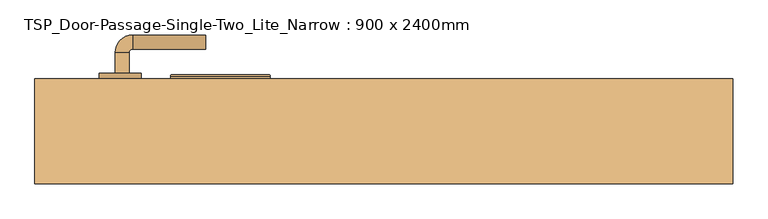
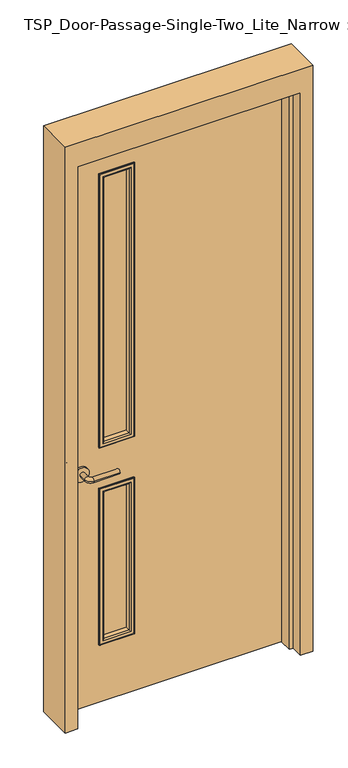
"""IFC4 building model written with IfcOpenShell, lengths in millimetres: door geometry, TSP_Door-Passage-Single-Two_Lite_Narrow : 900 x 2400mm."""

from ifc_helpers import new_model, si_unit, point, frame, frame_2d, origin, place, context, project, spatial, polyline, circle_curve, ellipse_curve, trimmed, segment, composite_curve, outline, extrude, faceted_brep, source, transform, mapped, element, save
from ifc_brep_helpers import plane_surface, cylinder_surface, revolved_surface, advanced_brep


def tsp_door_passage_single_two_lite_narrow_900_x_2400mm_46d0a56f(model_context):
    return source(origin(), model_context, "Body", "SolidModel", [
        advanced_brep(
        [(-384.990625, 48.35, 1000.0), (-364.990625, 48.35, 1000.0), (-364.990625, 18.35, 1000.0), (-384.990625, 18.35, 1000.0), (-359.990625, 13.35, 1000.0), (-359.990625, -6.65, 1000.0), (-254.990625, -6.65, 1000.0), (-254.990625, 13.35, 1000.0)],
        [
            (0, 1, circle_curve(frame((-374.990625, 48.35, 1000.0), z_axis=(0.0, 1.0, 0.0), x_axis=(1.0, 0.0, 0.0)), 10.0)),
            (1, 0, circle_curve(frame((-374.990625, 48.35, 1000.0), z_axis=(0.0, 1.0, 0.0), x_axis=(1.0, 0.0, 0.0)), 10.0)),
            (1, 2),
            (2, 3, circle_curve(frame((-374.990625, 18.35, 1000.0), z_axis=(0.0, 1.0, 0.0), x_axis=(1.0, 0.0, 0.0)), 10.0)),
            (3, 0),
            (3, 2, circle_curve(frame((-374.990625, 18.35, 1000.0), z_axis=(0.0, 1.0, 0.0), x_axis=(1.0, 0.0, 0.0)), 10.0)),
            (4, 5, circle_curve(frame((-359.990625, 3.35, 1000.0), z_axis=(-1.0, 0.0, 0.0), x_axis=(0.0, 1.0, 0.0)), 10.0)),
            (5, 3, circle_curve(frame((-359.990625, 18.35, 1000.0), z_axis=(0.0, 0.0, -1.0), x_axis=(-1.0, 0.0, 0.0)), 25.0)),
            (2, 4, circle_curve(frame((-359.990625, 18.35, 1000.0), z_axis=(0.0, 0.0, 1.0), x_axis=(-1.0, 0.0, 0.0)), 5.0)),
            (5, 4, circle_curve(frame((-359.990625, 3.35, 1000.0), z_axis=(-1.0, 0.0, 0.0), x_axis=(0.0, 1.0, 0.0)), 10.0)),
            (6, 7, circle_curve(frame((-254.990625, 3.35, 1000.0), z_axis=(1.0, 0.0, 0.0), x_axis=(0.0, 1.0, 0.0)), 10.0)),
            (7, 6, circle_curve(frame((-254.990625, 3.35, 1000.0), z_axis=(1.0, 0.0, 0.0), x_axis=(0.0, 1.0, 0.0)), 10.0)),
            (4, 7),
            (6, 5),
        ],
        [
            plane_surface(frame((-374.990625, 48.35, 1000.0), z_axis=(0.0, 1.0, 0.0), x_axis=(0.0, 0.0, 1.0))),
            cylinder_surface(frame((-374.990625, 48.35, 1000.0), z_axis=(0.0, 1.0, 0.0), x_axis=(1.0, 0.0, 0.0)), 10.0),
            revolved_surface(trimmed(ellipse_curve(frame((-374.990625, 18.35, 1000.0), z_axis=(0.0, -1.0, 0.0), x_axis=(1.0, 0.0, 0.0)), 10.0, 10.0), [point((-384.990625, 18.35, 1000.0))], [point((-364.990625, 18.35, 1000.0))], True, "CARTESIAN"), (-359.990625, 18.35, 1000.0), (0.0, 0.0, -1.0)),
            revolved_surface(trimmed(ellipse_curve(frame((-374.990625, 18.35, 1000.0), z_axis=(0.0, -1.0, 0.0), x_axis=(1.0, 0.0, 0.0)), 10.0, 10.0), [point((-364.990625, 18.35, 1000.0))], [point((-384.990625, 18.35, 1000.0))], True, "CARTESIAN"), (-359.990625, 18.35, 1000.0), (0.0, 0.0, -1.0)),
            plane_surface(frame((-254.990625, 3.35, 1000.0), z_axis=(1.0, 0.0, 0.0), x_axis=(0.0, 0.0, 1.0))),
            cylinder_surface(frame((-359.990625, 3.35, 1000.0), z_axis=(-1.0, 0.0, 0.0), x_axis=(0.0, 1.0, 0.0)), 10.0),
        ],
        [
            (0, [[1, 2]]),
            (1, [[3, 4, 5, -2]]),
            (1, [[-5, 6, -3, -1]]),
            (2, [[7, 8, -4, 9]]),
            (3, [[10, -9, -6, -8]]),
            (4, [[11, 12]]),
            (5, [[13, -11, 14, -7]]),
            (5, [[-14, -12, -13, -10]]),
        ],
    ),
        extrude(outline(composite_curve([segment(trimmed(circle_curve(frame_2d((1000.0, -377.490625)), 30.0), [point((1000.0, -407.490625))], [point((1000.0, -347.490625))], False, "CARTESIAN"), True, "CONTINUOUS"), segment(trimmed(circle_curve(frame_2d((1000.0, -377.490625)), 30.0), [point((1000.0, -347.490625))], [point((1000.0, -407.490625))], False, "CARTESIAN"), True, "CONTINUOUS")], self_intersect=False)), frame((0.0, 48.35, 0.0), z_axis=(0.0, 1.0, 0.0), x_axis=(0.0, 0.0, 1.0)), (0.0, 0.0, 1.0), 8.0),
        advanced_brep(
        [(-384.990625, 109.35, 1000.0), (-364.990625, 109.35, 1000.0), (-384.990625, 139.35, 1000.0), (-364.990625, 139.35, 1000.0), (-359.990625, 144.35, 1000.0), (-359.990625, 164.35, 1000.0), (-254.990625, 164.35, 1000.0), (-254.990625, 144.35, 1000.0)],
        [
            (0, 1, circle_curve(frame((-374.990625, 109.35, 1000.0), z_axis=(0.0, -1.0, 0.0), x_axis=(1.0, 0.0, 0.0)), 10.0)),
            (1, 0, circle_curve(frame((-374.990625, 109.35, 1000.0), z_axis=(0.0, -1.0, 0.0), x_axis=(1.0, 0.0, 0.0)), 10.0)),
            (0, 2),
            (2, 3, circle_curve(frame((-374.990625, 139.35, 1000.0), z_axis=(0.0, -1.0, 0.0), x_axis=(1.0, 0.0, 0.0)), 10.0)),
            (3, 1),
            (3, 2, circle_curve(frame((-374.990625, 139.35, 1000.0), z_axis=(0.0, -1.0, 0.0), x_axis=(1.0, 0.0, 0.0)), 10.0)),
            (4, 3, circle_curve(frame((-359.990625, 139.35, 1000.0), z_axis=(0.0, 0.0, 1.0), x_axis=(-1.0, 0.0, 0.0)), 5.0)),
            (2, 5, circle_curve(frame((-359.990625, 139.35, 1000.0), z_axis=(0.0, 0.0, -1.0), x_axis=(-1.0, 0.0, 0.0)), 25.0)),
            (5, 4, circle_curve(frame((-359.990625, 154.35, 1000.0), z_axis=(-1.0, 0.0, 0.0), x_axis=(0.0, -1.0, 0.0)), 10.0)),
            (4, 5, circle_curve(frame((-359.990625, 154.35, 1000.0), z_axis=(-1.0, 0.0, 0.0), x_axis=(0.0, -1.0, 0.0)), 10.0)),
            (6, 7, circle_curve(frame((-254.990625, 154.35, 1000.0), z_axis=(1.0, 0.0, 0.0), x_axis=(0.0, -1.0, 0.0)), 10.0)),
            (7, 6, circle_curve(frame((-254.990625, 154.35, 1000.0), z_axis=(1.0, 0.0, 0.0), x_axis=(0.0, -1.0, 0.0)), 10.0)),
            (5, 6),
            (7, 4),
        ],
        [
            plane_surface(frame((-374.990625, 109.35, 1000.0), z_axis=(0.0, -1.0, 0.0), x_axis=(0.0, 0.0, 1.0))),
            cylinder_surface(frame((-374.990625, 109.35, 1000.0), z_axis=(0.0, -1.0, 0.0), x_axis=(1.0, 0.0, 0.0)), 10.0),
            revolved_surface(trimmed(ellipse_curve(frame((-374.990625, 139.35, 1000.0), z_axis=(0.0, -1.0, 0.0), x_axis=(1.0, 0.0, 0.0)), 10.0, 10.0), [point((-384.990625, 139.35, 1000.0))], [point((-364.990625, 139.35, 1000.0))], True, "CARTESIAN"), (-359.990625, 139.35, 1000.0), (0.0, 0.0, -1.0)),
            revolved_surface(trimmed(ellipse_curve(frame((-374.990625, 139.35, 1000.0), z_axis=(0.0, -1.0, 0.0), x_axis=(1.0, 0.0, 0.0)), 10.0, 10.0), [point((-364.990625, 139.35, 1000.0))], [point((-384.990625, 139.35, 1000.0))], True, "CARTESIAN"), (-359.990625, 139.35, 1000.0), (0.0, 0.0, -1.0)),
            plane_surface(frame((-254.990625, 154.35, 1000.0), z_axis=(1.0, 0.0, 0.0), x_axis=(0.0, 0.0, 1.0))),
            cylinder_surface(frame((-359.990625, 154.35, 1000.0), z_axis=(-1.0, 0.0, 0.0), x_axis=(0.0, -1.0, 0.0)), 10.0),
        ],
        [
            (0, [[1, 2]]),
            (1, [[-1, 3, 4, 5]]),
            (1, [[-2, -5, 6, -3]]),
            (2, [[7, -4, 8, 9]]),
            (3, [[-8, -6, -7, 10]]),
            (4, [[11, 12]]),
            (5, [[-9, 13, -12, 14]]),
            (5, [[-10, -14, -11, -13]]),
        ],
    ),
        extrude(outline(composite_curve([segment(trimmed(circle_curve(frame_2d((1000.0, -377.490625)), 30.0), [point((1000.0, -407.490625))], [point((1000.0, -347.490625))], False, "CARTESIAN"), True, "CONTINUOUS"), segment(trimmed(circle_curve(frame_2d((1000.0, -377.490625)), 30.0), [point((1000.0, -347.490625))], [point((1000.0, -407.490625))], False, "CARTESIAN"), True, "CONTINUOUS")], self_intersect=False)), frame((0.0, 101.35, 0.0), z_axis=(0.0, 1.0, 0.0), x_axis=(0.0, 0.0, 1.0)), (0.0, 0.0, 1.0), 8.0),
        extrude(outline(polyline([(2400.0, -450.0), (0.0, -450.0), (0.0, 450.0), (2400.0, 450.0), (2400.0, -450.0)]), holes=[polyline([(2247.6, -297.6), (2247.6, -170.6), (1095.25, -170.6), (1095.25, -297.6), (2247.6, -297.6)]), polyline([(904.75, -297.6), (904.75, -170.6), (254.0, -170.6), (254.0, -297.6), (904.75, -297.6)])]), frame((0.0, 56.35, 0.0), z_axis=(0.0, 1.0, 0.0), x_axis=(0.0, 0.0, 1.0)), (0.0, 0.0, 1.0), 45.0),
        faceted_brep([(450.0, 51.5875, 0.0), (450.0, 101.35, 0.0), (500.0, 101.35, 0.0), (500.0, -48.65, 0.0), (450.0, -48.65, 0.0), (450.0, 0.5625, 0.0), (434.125, 0.5625, 0.0), (434.125, 51.5875, 0.0), (450.0, 51.5875, 2400.0), (450.0, 101.35, 2400.0), (-450.0, 101.35, 2400.0), (-450.0, 101.35, 0.0), (-500.0, 101.35, 0.0), (-500.0, 101.35, 2500.0), (500.0, 101.35, 2500.0), (500.0, -48.65, 2500.0), (-500.0, -48.65, 2500.0), (-500.0, -48.65, 0.0), (-450.0, -48.65, 0.0), (-450.0, -48.65, 2400.0), (450.0, -48.65, 2400.0), (450.0, 0.5625, 2400.0), (-450.0, 0.5625, 2400.0), (-450.0, 0.5625, 0.0), (-434.125, 0.5625, 0.0), (-434.125, 0.5625, 2384.125), (434.125, 0.5625, 2384.125), (434.125, 51.5875, 2384.125), (-434.125, 51.5875, 2384.125), (-434.125, 51.5875, 0.0), (-450.0, 51.5875, 0.0), (-450.0, 51.5875, 2400.0)], [[[0, 1, 2, 3, 4, 5, 6, 7]], [[1, 0, 8, 9]], [[2, 1, 9, 10, 11, 12, 13, 14]], [[3, 2, 14, 15]], [[4, 3, 15, 16, 17, 18, 19, 20]], [[5, 4, 20, 21]], [[6, 5, 21, 22, 23, 24, 25, 26]], [[7, 6, 26, 27]], [[0, 7, 27, 28, 29, 30, 31, 8]], [[9, 8, 31, 10]], [[20, 19, 22, 21]], [[26, 25, 28, 27]], [[12, 11, 30, 29, 24, 23, 18, 17]], [[11, 10, 31, 30]], [[13, 12, 17, 16]], [[19, 18, 23, 22]], [[25, 24, 29, 28]], [[15, 14, 13, 16]]]),
        extrude(outline(polyline([(-170.6, 75.675), (-297.6, 75.675), (-297.6, 82.025), (-170.6, 82.025), (-170.6, 75.675)])), frame((0.0, 0.0, 1095.25), z_axis=(0.0, 0.0, 1.0), x_axis=(1.0, 0.0, 0.0)), (0.0, 0.0, 1.0), 1152.35),
        extrude(outline(polyline([(-170.6, 75.675), (-297.6, 75.675), (-297.6, 82.025), (-170.6, 82.025), (-170.6, 75.675)])), frame((0.0, 0.0, 254.0), z_axis=(0.0, 0.0, 1.0), x_axis=(1.0, 0.0, 0.0)), (0.0, 0.0, 1.0), 650.75),
        advanced_brep(
        [(-297.6, 82.3, 2247.6), (-297.6, 101.35, 2247.6), (-297.6, 101.35, 1095.25), (-297.6, 82.3, 1095.25), (-285.6, 102.35, 2235.6), (-285.6, 82.3, 2235.6), (-285.6, 82.3, 1107.25), (-285.6, 102.35, 1107.25), (-290.6, 107.35, 2240.6), (-290.6, 107.35, 1102.25), (-305.6, 105.35, 2255.6), (-303.6, 107.35, 2253.6), (-303.6, 107.35, 1089.25), (-305.6, 105.35, 1087.25), (-305.6, 101.35, 2255.6), (-305.6, 101.35, 1087.25), (-170.6, 101.35, 1095.25), (-170.6, 82.3, 1095.25), (-182.6, 82.3, 1107.25), (-182.6, 102.35, 1107.25), (-177.6, 107.35, 1102.25), (-164.6, 107.35, 1089.25), (-162.6, 105.35, 1087.25), (-162.6, 101.35, 1087.25), (-170.6, 101.35, 2247.6), (-170.6, 82.3, 2247.6), (-182.6, 82.3, 2235.6), (-182.6, 102.35, 2235.6), (-177.6, 107.35, 2240.6), (-164.6, 107.35, 2253.6), (-162.6, 105.35, 2255.6), (-162.6, 101.35, 2255.6)],
        [
            (0, 1),
            (1, 2),
            (2, 3),
            (3, 0),
            (4, 5),
            (5, 6),
            (6, 7),
            (7, 4),
            (8, 4, ellipse_curve(frame((-290.6, 102.35, 2240.6), z_axis=(-0.7071067811865475, 0.0, -0.7071067811865475), x_axis=(-0.7071067811865474, 0.0, 0.7071067811865476)), 7.0710678, 5.0)),
            (7, 9, ellipse_curve(frame((-290.6, 102.35, 1102.25), z_axis=(-0.7071067811865475, 0.0, 0.7071067811865475), x_axis=(0.7071067811865474, 0.0, 0.7071067811865476)), 7.0710678, 5.0)),
            (9, 8),
            (10, 11, ellipse_curve(frame((-303.6, 105.35, 2253.6), z_axis=(-0.7071067811865475, 0.0, -0.7071067811865475), x_axis=(-0.7071067811865474, 0.0, 0.7071067811865476)), 2.8284271, 2.0)),
            (11, 12),
            (12, 13, ellipse_curve(frame((-303.6, 105.35, 1089.25), z_axis=(-0.7071067811865475, 0.0, 0.7071067811865475), x_axis=(0.7071067811865474, 0.0, 0.7071067811865476)), 2.8284271, 2.0)),
            (13, 10),
            (14, 10),
            (13, 15),
            (15, 14),
            (2, 16),
            (16, 17),
            (17, 3),
            (6, 18),
            (18, 19),
            (19, 7),
            (19, 20, ellipse_curve(frame((-177.6, 102.35, 1102.25), z_axis=(-0.7071067811865475, 0.0, -0.7071067811865475), x_axis=(-0.7071067811865476, 0.0, 0.7071067811865474)), 7.0710678, 5.0)),
            (20, 9),
            (12, 21),
            (21, 22, ellipse_curve(frame((-164.6, 105.35, 1089.25), z_axis=(-0.7071067811865475, 0.0, -0.7071067811865475), x_axis=(-0.7071067811865476, 0.0, 0.7071067811865474)), 2.8284271, 2.0)),
            (22, 13),
            (22, 23),
            (23, 15),
            (16, 24),
            (24, 25),
            (25, 17),
            (18, 26),
            (26, 27),
            (27, 19),
            (27, 28, ellipse_curve(frame((-177.6, 102.35, 2240.6), z_axis=(0.7071067811865475, 0.0, -0.7071067811865475), x_axis=(-0.7071067811865474, 0.0, -0.7071067811865476)), 7.0710678, 5.0)),
            (28, 20),
            (21, 29),
            (29, 30, ellipse_curve(frame((-164.6, 105.35, 2253.6), z_axis=(0.7071067811865475, 0.0, -0.7071067811865475), x_axis=(-0.7071067811865474, 0.0, -0.7071067811865476)), 2.8284271, 2.0)),
            (30, 22),
            (30, 31),
            (31, 23),
            (31, 14),
            (1, 24),
            (0, 25),
            (5, 26),
            (4, 27),
            (8, 28),
            (11, 29),
            (10, 30),
        ],
        [
            plane_surface(frame((-297.6, 101.35, 2247.6), z_axis=(-1.0, 0.0, 0.0), x_axis=(0.0, 0.0, -1.0))),
            plane_surface(frame((-285.6, 82.3, 2235.6), z_axis=(1.0, 0.0, 0.0), x_axis=(0.0, 0.0, -1.0))),
            cylinder_surface(frame((-290.6, 102.35, 2247.6), z_axis=(0.0, 0.0, 1.0), x_axis=(-1.0, 0.0, 0.0)), 5.0),
            cylinder_surface(frame((-303.6, 105.35, 2247.6), z_axis=(0.0, 0.0, 1.0), x_axis=(-1.0, 0.0, 0.0)), 2.0),
            plane_surface(frame((-305.6, 105.35, 2255.6), z_axis=(-1.0, 0.0, 0.0), x_axis=(0.0, 0.0, -1.0))),
            plane_surface(frame((-297.6, 101.35, 1095.25), z_axis=(0.0, 0.0, -1.0), x_axis=(1.0, 0.0, 0.0))),
            plane_surface(frame((-285.6, 82.3, 1107.25), z_axis=(0.0, 0.0, 1.0), x_axis=(1.0, 0.0, 0.0))),
            cylinder_surface(frame((-297.6, 102.35, 1102.25), z_axis=(-1.0, 0.0, 0.0), x_axis=(0.0, 0.0, -1.0)), 5.0),
            cylinder_surface(frame((-297.6, 105.35, 1089.25), z_axis=(-1.0, 0.0, 0.0), x_axis=(0.0, 0.0, -1.0)), 2.0),
            plane_surface(frame((-305.6, 105.35, 1087.25), z_axis=(0.0, 0.0, -1.0), x_axis=(1.0, 0.0, 0.0))),
            plane_surface(frame((-170.6, 101.35, 1095.25), z_axis=(1.0, 0.0, 0.0), x_axis=(0.0, 0.0, 1.0))),
            plane_surface(frame((-182.6, 82.3, 1107.25), z_axis=(-1.0, 0.0, 0.0), x_axis=(0.0, 0.0, 1.0))),
            cylinder_surface(frame((-177.6, 102.35, 1095.25), z_axis=(0.0, 0.0, -1.0), x_axis=(1.0, 0.0, 0.0)), 5.0),
            cylinder_surface(frame((-164.6, 105.35, 1095.25), z_axis=(0.0, 0.0, -1.0), x_axis=(1.0, 0.0, 0.0)), 2.0),
            plane_surface(frame((-162.6, 105.35, 1087.25), z_axis=(1.0, 0.0, 0.0), x_axis=(0.0, 0.0, 1.0))),
            plane_surface(frame((-162.6, 101.35, 2255.6), z_axis=(0.0, -1.0, 0.0), x_axis=(-1.0, 0.0, 0.0))),
            plane_surface(frame((-170.6, 101.35, 2247.6), z_axis=(0.0, 0.0, 1.0), x_axis=(-1.0, 0.0, 0.0))),
            plane_surface(frame((-170.6, 82.3, 2247.6), z_axis=(0.0, -1.0, 0.0), x_axis=(-1.0, 0.0, 0.0))),
            plane_surface(frame((-182.6, 82.3, 2235.6), z_axis=(0.0, 0.0, -1.0), x_axis=(-1.0, 0.0, 0.0))),
            cylinder_surface(frame((-170.6, 102.35, 2240.6), z_axis=(1.0, 0.0, 0.0), x_axis=(0.0, 0.0, 1.0)), 5.0),
            plane_surface(frame((-177.6, 107.35, 2240.6), z_axis=(0.0, 1.0, 0.0), x_axis=(-1.0, 0.0, 0.0))),
            cylinder_surface(frame((-170.6, 105.35, 2253.6), z_axis=(1.0, 0.0, 0.0), x_axis=(0.0, 0.0, 1.0)), 2.0),
            plane_surface(frame((-162.6, 105.35, 2255.6), z_axis=(0.0, 0.0, 1.0), x_axis=(-1.0, 0.0, 0.0))),
        ],
        [
            (0, [[1, 2, 3, 4]]),
            (1, [[5, 6, 7, 8]]),
            (2, [[9, -8, 10, 11]]),
            (3, [[12, 13, 14, 15]]),
            (4, [[16, -15, 17, 18]]),
            (5, [[-3, 19, 20, 21]]),
            (6, [[-7, 22, 23, 24]]),
            (7, [[-10, -24, 25, 26]]),
            (8, [[-14, 27, 28, 29]]),
            (9, [[-17, -29, 30, 31]]),
            (10, [[-20, 32, 33, 34]]),
            (11, [[-23, 35, 36, 37]]),
            (12, [[-25, -37, 38, 39]]),
            (13, [[-28, 40, 41, 42]]),
            (14, [[-30, -42, 43, 44]]),
            (15, [[-31, -44, 45, -18], [46, -32, -19, -2]]),
            (16, [[-33, -46, -1, 47]]),
            (17, [[-21, -34, -47, -4], [48, -35, -22, -6]]),
            (18, [[-36, -48, -5, 49]]),
            (19, [[-38, -49, -9, 50]]),
            (20, [[51, -40, -27, -13], [-26, -39, -50, -11]]),
            (21, [[-41, -51, -12, 52]]),
            (22, [[-43, -52, -16, -45]]),
        ],
    ),
        advanced_brep(
        [(-297.6, 75.4, 1095.25), (-297.6, 56.35, 1095.25), (-297.6, 56.35, 2247.6), (-297.6, 75.4, 2247.6), (-285.6, 55.35, 1107.25), (-285.6, 75.4, 1107.25), (-285.6, 75.4, 2235.6), (-285.6, 55.35, 2235.6), (-290.6, 50.35, 1102.25), (-290.6, 50.35, 2240.6), (-305.6, 52.35, 1087.25), (-303.6, 50.35, 1089.25), (-303.6, 50.35, 2253.6), (-305.6, 52.35, 2255.6), (-305.6, 56.35, 1087.25), (-305.6, 56.35, 2255.6), (-170.6, 56.35, 2247.6), (-170.6, 75.4, 2247.6), (-182.6, 75.4, 2235.6), (-182.6, 55.35, 2235.6), (-177.6, 50.35, 2240.6), (-164.6, 50.35, 2253.6), (-162.6, 52.35, 2255.6), (-162.6, 56.35, 2255.6), (-170.6, 56.35, 1095.25), (-170.6, 75.4, 1095.25), (-182.6, 75.4, 1107.25), (-182.6, 55.35, 1107.25), (-177.6, 50.35, 1102.25), (-164.6, 50.35, 1089.25), (-162.6, 52.35, 1087.25), (-162.6, 56.35, 1087.25)],
        [
            (0, 1),
            (1, 2),
            (2, 3),
            (3, 0),
            (4, 5),
            (5, 6),
            (6, 7),
            (7, 4),
            (8, 4, ellipse_curve(frame((-290.6, 55.35, 1102.25), z_axis=(-0.7071067811865475, 0.0, 0.7071067811865475), x_axis=(-0.7071067811865474, 0.0, -0.7071067811865476)), 7.0710678, 5.0)),
            (7, 9, ellipse_curve(frame((-290.6, 55.35, 2240.6), z_axis=(-0.7071067811865475, 0.0, -0.7071067811865475), x_axis=(0.7071067811865474, 0.0, -0.7071067811865476)), 7.0710678, 5.0)),
            (9, 8),
            (10, 11, ellipse_curve(frame((-303.6, 52.35, 1089.25), z_axis=(-0.7071067811865475, 0.0, 0.7071067811865475), x_axis=(-0.7071067811865474, 0.0, -0.7071067811865476)), 2.8284271, 2.0)),
            (11, 12),
            (12, 13, ellipse_curve(frame((-303.6, 52.35, 2253.6), z_axis=(-0.7071067811865475, 0.0, -0.7071067811865475), x_axis=(0.7071067811865474, 0.0, -0.7071067811865476)), 2.8284271, 2.0)),
            (13, 10),
            (14, 10),
            (13, 15),
            (15, 14),
            (2, 16),
            (16, 17),
            (17, 3),
            (6, 18),
            (18, 19),
            (19, 7),
            (19, 20, ellipse_curve(frame((-177.6, 55.35, 2240.6), z_axis=(-0.7071067811865475, 0.0, 0.7071067811865475), x_axis=(-0.7071067811865476, 0.0, -0.7071067811865474)), 7.0710678, 5.0)),
            (20, 9),
            (12, 21),
            (21, 22, ellipse_curve(frame((-164.6, 52.35, 2253.6), z_axis=(-0.7071067811865475, 0.0, 0.7071067811865475), x_axis=(-0.7071067811865476, 0.0, -0.7071067811865474)), 2.8284271, 2.0)),
            (22, 13),
            (22, 23),
            (23, 15),
            (16, 24),
            (24, 25),
            (25, 17),
            (18, 26),
            (26, 27),
            (27, 19),
            (27, 28, ellipse_curve(frame((-177.6, 55.35, 1102.25), z_axis=(0.7071067811865475, 0.0, 0.7071067811865475), x_axis=(-0.7071067811865474, 0.0, 0.7071067811865476)), 7.0710678, 5.0)),
            (28, 20),
            (21, 29),
            (29, 30, ellipse_curve(frame((-164.6, 52.35, 1089.25), z_axis=(0.7071067811865475, 0.0, 0.7071067811865475), x_axis=(-0.7071067811865474, 0.0, 0.7071067811865476)), 2.8284271, 2.0)),
            (30, 22),
            (30, 31),
            (31, 23),
            (31, 14),
            (1, 24),
            (0, 25),
            (5, 26),
            (4, 27),
            (8, 28),
            (11, 29),
            (10, 30),
        ],
        [
            plane_surface(frame((-297.6, 56.35, 1095.25), z_axis=(-1.0, 0.0, 0.0), x_axis=(0.0, 0.0, 1.0))),
            plane_surface(frame((-285.6, 75.4, 1107.25), z_axis=(1.0, 0.0, 0.0), x_axis=(0.0, 0.0, 1.0))),
            cylinder_surface(frame((-290.6, 55.35, 1095.25), z_axis=(0.0, 0.0, -1.0), x_axis=(-1.0, 0.0, 0.0)), 5.0),
            cylinder_surface(frame((-303.6, 52.35, 1095.25), z_axis=(0.0, 0.0, -1.0), x_axis=(-1.0, 0.0, 0.0)), 2.0),
            plane_surface(frame((-305.6, 52.35, 1087.25), z_axis=(-1.0, 0.0, 0.0), x_axis=(0.0, 0.0, 1.0))),
            plane_surface(frame((-297.6, 56.35, 2247.6), z_axis=(0.0, 0.0, 1.0), x_axis=(1.0, 0.0, 0.0))),
            plane_surface(frame((-285.6, 75.4, 2235.6), z_axis=(0.0, 0.0, -1.0), x_axis=(1.0, 0.0, 0.0))),
            cylinder_surface(frame((-297.6, 55.35, 2240.6), z_axis=(-1.0, 0.0, 0.0), x_axis=(0.0, 0.0, 1.0)), 5.0),
            cylinder_surface(frame((-297.6, 52.35, 2253.6), z_axis=(-1.0, 0.0, 0.0), x_axis=(0.0, 0.0, 1.0)), 2.0),
            plane_surface(frame((-305.6, 52.35, 2255.6), z_axis=(0.0, 0.0, 1.0), x_axis=(1.0, 0.0, 0.0))),
            plane_surface(frame((-170.6, 56.35, 2247.6), z_axis=(1.0, 0.0, 0.0), x_axis=(0.0, 0.0, -1.0))),
            plane_surface(frame((-182.6, 75.4, 2235.6), z_axis=(-1.0, 0.0, 0.0), x_axis=(0.0, 0.0, -1.0))),
            cylinder_surface(frame((-177.6, 55.35, 2247.6), z_axis=(0.0, 0.0, 1.0), x_axis=(1.0, 0.0, 0.0)), 5.0),
            cylinder_surface(frame((-164.6, 52.35, 2247.6), z_axis=(0.0, 0.0, 1.0), x_axis=(1.0, 0.0, 0.0)), 2.0),
            plane_surface(frame((-162.6, 52.35, 2255.6), z_axis=(1.0, 0.0, 0.0), x_axis=(0.0, 0.0, -1.0))),
            plane_surface(frame((-162.6, 56.35, 1087.25), z_axis=(0.0, 1.0, 0.0), x_axis=(-1.0, 0.0, 0.0))),
            plane_surface(frame((-170.6, 56.35, 1095.25), z_axis=(0.0, 0.0, -1.0), x_axis=(-1.0, 0.0, 0.0))),
            plane_surface(frame((-170.6, 75.4, 1095.25), z_axis=(0.0, 1.0, 0.0), x_axis=(-1.0, 0.0, 0.0))),
            plane_surface(frame((-182.6, 75.4, 1107.25), z_axis=(0.0, 0.0, 1.0), x_axis=(-1.0, 0.0, 0.0))),
            cylinder_surface(frame((-170.6, 55.35, 1102.25), z_axis=(1.0, 0.0, 0.0), x_axis=(0.0, 0.0, -1.0)), 5.0),
            plane_surface(frame((-177.6, 50.35, 1102.25), z_axis=(0.0, -1.0, 0.0), x_axis=(-1.0, 0.0, 0.0))),
            cylinder_surface(frame((-170.6, 52.35, 1089.25), z_axis=(1.0, 0.0, 0.0), x_axis=(0.0, 0.0, -1.0)), 2.0),
            plane_surface(frame((-162.6, 52.35, 1087.25), z_axis=(0.0, 0.0, -1.0), x_axis=(-1.0, 0.0, 0.0))),
        ],
        [
            (0, [[1, 2, 3, 4]]),
            (1, [[5, 6, 7, 8]]),
            (2, [[9, -8, 10, 11]]),
            (3, [[12, 13, 14, 15]]),
            (4, [[16, -15, 17, 18]]),
            (5, [[-3, 19, 20, 21]]),
            (6, [[-7, 22, 23, 24]]),
            (7, [[-10, -24, 25, 26]]),
            (8, [[-14, 27, 28, 29]]),
            (9, [[-17, -29, 30, 31]]),
            (10, [[-20, 32, 33, 34]]),
            (11, [[-23, 35, 36, 37]]),
            (12, [[-25, -37, 38, 39]]),
            (13, [[-28, 40, 41, 42]]),
            (14, [[-30, -42, 43, 44]]),
            (15, [[-31, -44, 45, -18], [46, -32, -19, -2]]),
            (16, [[-33, -46, -1, 47]]),
            (17, [[-21, -34, -47, -4], [48, -35, -22, -6]]),
            (18, [[-36, -48, -5, 49]]),
            (19, [[-38, -49, -9, 50]]),
            (20, [[51, -40, -27, -13], [-26, -39, -50, -11]]),
            (21, [[-41, -51, -12, 52]]),
            (22, [[-43, -52, -16, -45]]),
        ],
    ),
        advanced_brep(
        [(-297.6, 82.3, 904.75), (-297.6, 101.35, 904.75), (-297.6, 101.35, 254.0), (-297.6, 82.3, 254.0), (-285.6, 102.35, 892.75), (-285.6, 82.3, 892.75), (-285.6, 82.3, 266.0), (-285.6, 102.35, 266.0), (-290.6, 107.35, 897.75), (-290.6, 107.35, 261.0), (-305.6, 105.35, 912.75), (-303.6, 107.35, 910.75), (-303.6, 107.35, 248.0), (-305.6, 105.35, 246.0), (-305.6, 101.35, 912.75), (-305.6, 101.35, 246.0), (-170.6, 101.35, 254.0), (-170.6, 82.3, 254.0), (-182.6, 82.3, 266.0), (-182.6, 102.35, 266.0), (-177.6, 107.35, 261.0), (-164.6, 107.35, 248.0), (-162.6, 105.35, 246.0), (-162.6, 101.35, 246.0), (-170.6, 101.35, 904.75), (-170.6, 82.3, 904.75), (-182.6, 82.3, 892.75), (-182.6, 102.35, 892.75), (-177.6, 107.35, 897.75), (-164.6, 107.35, 910.75), (-162.6, 105.35, 912.75), (-162.6, 101.35, 912.75)],
        [
            (0, 1),
            (1, 2),
            (2, 3),
            (3, 0),
            (4, 5),
            (5, 6),
            (6, 7),
            (7, 4),
            (8, 4, ellipse_curve(frame((-290.6, 102.35, 897.75), z_axis=(-0.7071067811865475, 0.0, -0.7071067811865475), x_axis=(-0.7071067811865474, 0.0, 0.7071067811865476)), 7.0710678, 5.0)),
            (7, 9, ellipse_curve(frame((-290.6, 102.35, 261.0), z_axis=(-0.7071067811865475, 0.0, 0.7071067811865475), x_axis=(0.7071067811865474, 0.0, 0.7071067811865476)), 7.0710678, 5.0)),
            (9, 8),
            (10, 11, ellipse_curve(frame((-303.6, 105.35, 910.75), z_axis=(-0.7071067811865475, 0.0, -0.7071067811865475), x_axis=(-0.7071067811865474, 0.0, 0.7071067811865476)), 2.8284271, 2.0)),
            (11, 12),
            (12, 13, ellipse_curve(frame((-303.6, 105.35, 248.0), z_axis=(-0.7071067811865475, 0.0, 0.7071067811865475), x_axis=(0.7071067811865474, 0.0, 0.7071067811865476)), 2.8284271, 2.0)),
            (13, 10),
            (14, 10),
            (13, 15),
            (15, 14),
            (2, 16),
            (16, 17),
            (17, 3),
            (6, 18),
            (18, 19),
            (19, 7),
            (19, 20, ellipse_curve(frame((-177.6, 102.35, 261.0), z_axis=(-0.7071067811865475, 0.0, -0.7071067811865475), x_axis=(-0.7071067811865476, 0.0, 0.7071067811865474)), 7.0710678, 5.0)),
            (20, 9),
            (12, 21),
            (21, 22, ellipse_curve(frame((-164.6, 105.35, 248.0), z_axis=(-0.7071067811865475, 0.0, -0.7071067811865475), x_axis=(-0.7071067811865476, 0.0, 0.7071067811865474)), 2.8284271, 2.0)),
            (22, 13),
            (22, 23),
            (23, 15),
            (16, 24),
            (24, 25),
            (25, 17),
            (18, 26),
            (26, 27),
            (27, 19),
            (27, 28, ellipse_curve(frame((-177.6, 102.35, 897.75), z_axis=(0.7071067811865475, 0.0, -0.7071067811865475), x_axis=(-0.7071067811865474, 0.0, -0.7071067811865476)), 7.0710678, 5.0)),
            (28, 20),
            (21, 29),
            (29, 30, ellipse_curve(frame((-164.6, 105.35, 910.75), z_axis=(0.7071067811865475, 0.0, -0.7071067811865475), x_axis=(-0.7071067811865474, 0.0, -0.7071067811865476)), 2.8284271, 2.0)),
            (30, 22),
            (30, 31),
            (31, 23),
            (31, 14),
            (1, 24),
            (0, 25),
            (5, 26),
            (4, 27),
            (8, 28),
            (11, 29),
            (10, 30),
        ],
        [
            plane_surface(frame((-297.6, 101.35, 904.75), z_axis=(-1.0, 0.0, 0.0), x_axis=(0.0, 0.0, -1.0))),
            plane_surface(frame((-285.6, 82.3, 892.75), z_axis=(1.0, 0.0, 0.0), x_axis=(0.0, 0.0, -1.0))),
            cylinder_surface(frame((-290.6, 102.35, 904.75), z_axis=(0.0, 0.0, 1.0), x_axis=(-1.0, 0.0, 0.0)), 5.0),
            cylinder_surface(frame((-303.6, 105.35, 904.75), z_axis=(0.0, 0.0, 1.0), x_axis=(-1.0, 0.0, 0.0)), 2.0),
            plane_surface(frame((-305.6, 105.35, 912.75), z_axis=(-1.0, 0.0, 0.0), x_axis=(0.0, 0.0, -1.0))),
            plane_surface(frame((-297.6, 101.35, 254.0), z_axis=(0.0, 0.0, -1.0), x_axis=(1.0, 0.0, 0.0))),
            plane_surface(frame((-285.6, 82.3, 266.0), z_axis=(0.0, 0.0, 1.0), x_axis=(1.0, 0.0, 0.0))),
            cylinder_surface(frame((-297.6, 102.35, 261.0), z_axis=(-1.0, 0.0, 0.0), x_axis=(0.0, 0.0, -1.0)), 5.0),
            cylinder_surface(frame((-297.6, 105.35, 248.0), z_axis=(-1.0, 0.0, 0.0), x_axis=(0.0, 0.0, -1.0)), 2.0),
            plane_surface(frame((-305.6, 105.35, 246.0), z_axis=(0.0, 0.0, -1.0), x_axis=(1.0, 0.0, 0.0))),
            plane_surface(frame((-170.6, 101.35, 254.0), z_axis=(1.0, 0.0, 0.0), x_axis=(0.0, 0.0, 1.0))),
            plane_surface(frame((-182.6, 82.3, 266.0), z_axis=(-1.0, 0.0, 0.0), x_axis=(0.0, 0.0, 1.0))),
            cylinder_surface(frame((-177.6, 102.35, 254.0), z_axis=(0.0, 0.0, -1.0), x_axis=(1.0, 0.0, 0.0)), 5.0),
            cylinder_surface(frame((-164.6, 105.35, 254.0), z_axis=(0.0, 0.0, -1.0), x_axis=(1.0, 0.0, 0.0)), 2.0),
            plane_surface(frame((-162.6, 105.35, 246.0), z_axis=(1.0, 0.0, 0.0), x_axis=(0.0, 0.0, 1.0))),
            plane_surface(frame((-162.6, 101.35, 912.75), z_axis=(0.0, -1.0, 0.0), x_axis=(-1.0, 0.0, 0.0))),
            plane_surface(frame((-170.6, 101.35, 904.75), z_axis=(0.0, 0.0, 1.0), x_axis=(-1.0, 0.0, 0.0))),
            plane_surface(frame((-170.6, 82.3, 904.75), z_axis=(0.0, -1.0, 0.0), x_axis=(-1.0, 0.0, 0.0))),
            plane_surface(frame((-182.6, 82.3, 892.75), z_axis=(0.0, 0.0, -1.0), x_axis=(-1.0, 0.0, 0.0))),
            cylinder_surface(frame((-170.6, 102.35, 897.75), z_axis=(1.0, 0.0, 0.0), x_axis=(0.0, 0.0, 1.0)), 5.0),
            plane_surface(frame((-177.6, 107.35, 897.75), z_axis=(0.0, 1.0, 0.0), x_axis=(-1.0, 0.0, 0.0))),
            cylinder_surface(frame((-170.6, 105.35, 910.75), z_axis=(1.0, 0.0, 0.0), x_axis=(0.0, 0.0, 1.0)), 2.0),
            plane_surface(frame((-162.6, 105.35, 912.75), z_axis=(0.0, 0.0, 1.0), x_axis=(-1.0, 0.0, 0.0))),
        ],
        [
            (0, [[1, 2, 3, 4]]),
            (1, [[5, 6, 7, 8]]),
            (2, [[9, -8, 10, 11]]),
            (3, [[12, 13, 14, 15]]),
            (4, [[16, -15, 17, 18]]),
            (5, [[-3, 19, 20, 21]]),
            (6, [[-7, 22, 23, 24]]),
            (7, [[-10, -24, 25, 26]]),
            (8, [[-14, 27, 28, 29]]),
            (9, [[-17, -29, 30, 31]]),
            (10, [[-20, 32, 33, 34]]),
            (11, [[-23, 35, 36, 37]]),
            (12, [[-25, -37, 38, 39]]),
            (13, [[-28, 40, 41, 42]]),
            (14, [[-30, -42, 43, 44]]),
            (15, [[-31, -44, 45, -18], [46, -32, -19, -2]]),
            (16, [[-33, -46, -1, 47]]),
            (17, [[-21, -34, -47, -4], [48, -35, -22, -6]]),
            (18, [[-36, -48, -5, 49]]),
            (19, [[-38, -49, -9, 50]]),
            (20, [[51, -40, -27, -13], [-26, -39, -50, -11]]),
            (21, [[-41, -51, -12, 52]]),
            (22, [[-43, -52, -16, -45]]),
        ],
    ),
        advanced_brep(
        [(-170.6, 75.4, 904.75), (-170.6, 56.35, 904.75), (-170.6, 56.35, 254.0), (-170.6, 75.4, 254.0), (-182.6, 55.35, 892.75), (-182.6, 75.4, 892.75), (-182.6, 75.4, 266.0), (-182.6, 55.35, 266.0), (-177.6, 50.35, 897.75), (-177.6, 50.35, 261.0), (-162.6, 52.35, 912.75), (-164.6, 50.35, 910.75), (-164.6, 50.35, 248.0), (-162.6, 52.35, 246.0), (-162.6, 56.35, 912.75), (-162.6, 56.35, 246.0), (-297.6, 56.35, 254.0), (-297.6, 75.4, 254.0), (-285.6, 75.4, 266.0), (-285.6, 55.35, 266.0), (-290.6, 50.35, 261.0), (-303.6, 50.35, 248.0), (-305.6, 52.35, 246.0), (-305.6, 56.35, 246.0), (-297.6, 56.35, 904.75), (-297.6, 75.4, 904.75), (-285.6, 75.4, 892.75), (-285.6, 55.35, 892.75), (-290.6, 50.35, 897.75), (-303.6, 50.35, 910.75), (-305.6, 52.35, 912.75), (-305.6, 56.35, 912.75)],
        [
            (0, 1),
            (1, 2),
            (2, 3),
            (3, 0),
            (4, 5),
            (5, 6),
            (6, 7),
            (7, 4),
            (8, 4, ellipse_curve(frame((-177.6, 55.35, 897.75), z_axis=(0.7071067811865475, 0.0, -0.7071067811865475), x_axis=(0.7071067811865474, 0.0, 0.7071067811865476)), 7.0710678, 5.0)),
            (7, 9, ellipse_curve(frame((-177.6, 55.35, 261.0), z_axis=(0.7071067811865475, 0.0, 0.7071067811865475), x_axis=(-0.7071067811865474, 0.0, 0.7071067811865476)), 7.0710678, 5.0)),
            (9, 8),
            (10, 11, ellipse_curve(frame((-164.6, 52.35, 910.75), z_axis=(0.7071067811865475, 0.0, -0.7071067811865475), x_axis=(0.7071067811865474, 0.0, 0.7071067811865476)), 2.8284271, 2.0)),
            (11, 12),
            (12, 13, ellipse_curve(frame((-164.6, 52.35, 248.0), z_axis=(0.7071067811865475, 0.0, 0.7071067811865475), x_axis=(-0.7071067811865474, 0.0, 0.7071067811865476)), 2.8284271, 2.0)),
            (13, 10),
            (14, 10),
            (13, 15),
            (15, 14),
            (2, 16),
            (16, 17),
            (17, 3),
            (6, 18),
            (18, 19),
            (19, 7),
            (19, 20, ellipse_curve(frame((-290.6, 55.35, 261.0), z_axis=(0.7071067811865475, 0.0, -0.7071067811865475), x_axis=(0.7071067811865476, 0.0, 0.7071067811865474)), 7.0710678, 5.0)),
            (20, 9),
            (12, 21),
            (21, 22, ellipse_curve(frame((-303.6, 52.35, 248.0), z_axis=(0.7071067811865475, 0.0, -0.7071067811865475), x_axis=(0.7071067811865476, 0.0, 0.7071067811865474)), 2.8284271, 2.0)),
            (22, 13),
            (22, 23),
            (23, 15),
            (16, 24),
            (24, 25),
            (25, 17),
            (18, 26),
            (26, 27),
            (27, 19),
            (27, 28, ellipse_curve(frame((-290.6, 55.35, 897.75), z_axis=(-0.7071067811865475, 0.0, -0.7071067811865475), x_axis=(0.7071067811865474, 0.0, -0.7071067811865476)), 7.0710678, 5.0)),
            (28, 20),
            (21, 29),
            (29, 30, ellipse_curve(frame((-303.6, 52.35, 910.75), z_axis=(-0.7071067811865475, 0.0, -0.7071067811865475), x_axis=(0.7071067811865474, 0.0, -0.7071067811865476)), 2.8284271, 2.0)),
            (30, 22),
            (30, 31),
            (31, 23),
            (31, 14),
            (1, 24),
            (0, 25),
            (5, 26),
            (4, 27),
            (8, 28),
            (11, 29),
            (10, 30),
        ],
        [
            plane_surface(frame((-170.6, 56.35, 904.75), z_axis=(1.0, 0.0, 0.0), x_axis=(0.0, 0.0, -1.0))),
            plane_surface(frame((-182.6, 75.4, 892.75), z_axis=(-1.0, 0.0, 0.0), x_axis=(0.0, 0.0, -1.0))),
            cylinder_surface(frame((-177.6, 55.35, 904.75), z_axis=(0.0, 0.0, 1.0), x_axis=(1.0, 0.0, 0.0)), 5.0),
            cylinder_surface(frame((-164.6, 52.35, 904.75), z_axis=(0.0, 0.0, 1.0), x_axis=(1.0, 0.0, 0.0)), 2.0),
            plane_surface(frame((-162.6, 52.35, 912.75), z_axis=(1.0, 0.0, 0.0), x_axis=(0.0, 0.0, -1.0))),
            plane_surface(frame((-170.6, 56.35, 254.0), z_axis=(0.0, 0.0, -1.0), x_axis=(-1.0, 0.0, 0.0))),
            plane_surface(frame((-182.6, 75.4, 266.0), z_axis=(0.0, 0.0, 1.0), x_axis=(-1.0, 0.0, 0.0))),
            cylinder_surface(frame((-170.6, 55.35, 261.0), z_axis=(1.0, 0.0, 0.0), x_axis=(0.0, 0.0, -1.0)), 5.0),
            cylinder_surface(frame((-170.6, 52.35, 248.0), z_axis=(1.0, 0.0, 0.0), x_axis=(0.0, 0.0, -1.0)), 2.0),
            plane_surface(frame((-162.6, 52.35, 246.0), z_axis=(0.0, 0.0, -1.0), x_axis=(-1.0, 0.0, 0.0))),
            plane_surface(frame((-297.6, 56.35, 254.0), z_axis=(-1.0, 0.0, 0.0), x_axis=(0.0, 0.0, 1.0))),
            plane_surface(frame((-285.6, 75.4, 266.0), z_axis=(1.0, 0.0, 0.0), x_axis=(0.0, 0.0, 1.0))),
            cylinder_surface(frame((-290.6, 55.35, 254.0), z_axis=(0.0, 0.0, -1.0), x_axis=(-1.0, 0.0, 0.0)), 5.0),
            cylinder_surface(frame((-303.6, 52.35, 254.0), z_axis=(0.0, 0.0, -1.0), x_axis=(-1.0, 0.0, 0.0)), 2.0),
            plane_surface(frame((-305.6, 52.35, 246.0), z_axis=(-1.0, 0.0, 0.0), x_axis=(0.0, 0.0, 1.0))),
            plane_surface(frame((-305.6, 56.35, 912.75), z_axis=(0.0, 1.0, 0.0), x_axis=(1.0, 0.0, 0.0))),
            plane_surface(frame((-297.6, 56.35, 904.75), z_axis=(0.0, 0.0, 1.0), x_axis=(1.0, 0.0, 0.0))),
            plane_surface(frame((-297.6, 75.4, 904.75), z_axis=(0.0, 1.0, 0.0), x_axis=(1.0, 0.0, 0.0))),
            plane_surface(frame((-285.6, 75.4, 892.75), z_axis=(0.0, 0.0, -1.0), x_axis=(1.0, 0.0, 0.0))),
            cylinder_surface(frame((-297.6, 55.35, 897.75), z_axis=(-1.0, 0.0, 0.0), x_axis=(0.0, 0.0, 1.0)), 5.0),
            plane_surface(frame((-290.6, 50.35, 897.75), z_axis=(0.0, -1.0, 0.0), x_axis=(1.0, 0.0, 0.0))),
            cylinder_surface(frame((-297.6, 52.35, 910.75), z_axis=(-1.0, 0.0, 0.0), x_axis=(0.0, 0.0, 1.0)), 2.0),
            plane_surface(frame((-305.6, 52.35, 912.75), z_axis=(0.0, 0.0, 1.0), x_axis=(1.0, 0.0, 0.0))),
        ],
        [
            (0, [[1, 2, 3, 4]]),
            (1, [[5, 6, 7, 8]]),
            (2, [[9, -8, 10, 11]]),
            (3, [[12, 13, 14, 15]]),
            (4, [[16, -15, 17, 18]]),
            (5, [[-3, 19, 20, 21]]),
            (6, [[-7, 22, 23, 24]]),
            (7, [[-10, -24, 25, 26]]),
            (8, [[-14, 27, 28, 29]]),
            (9, [[-17, -29, 30, 31]]),
            (10, [[-20, 32, 33, 34]]),
            (11, [[-23, 35, 36, 37]]),
            (12, [[-25, -37, 38, 39]]),
            (13, [[-28, 40, 41, 42]]),
            (14, [[-30, -42, 43, 44]]),
            (15, [[-31, -44, 45, -18], [46, -32, -19, -2]]),
            (16, [[-33, -46, -1, 47]]),
            (17, [[-21, -34, -47, -4], [48, -35, -22, -6]]),
            (18, [[-36, -48, -5, 49]]),
            (19, [[-38, -49, -9, 50]]),
            (20, [[51, -40, -27, -13], [-26, -39, -50, -11]]),
            (21, [[-41, -51, -12, 52]]),
            (22, [[-43, -52, -16, -45]]),
        ],
    ),
    ])


if __name__ == "__main__":
    model = new_model("IFC4")
    model_context = context("Model", 3, world=origin())
    ifc_project = project(units=[si_unit("LENGTHUNIT", "METRE", prefix="MILLI")], contexts=[model_context])
    site = spatial("IfcSite", under=ifc_project)
    building = spatial("IfcBuilding", under=site)
    placement = place(None, origin())
    tsp_door_passage_single_two_lite_narrow_900_x_2400mm_shape = tsp_door_passage_single_two_lite_narrow_900_x_2400mm_46d0a56f(model_context)
    element("IfcDoor", 1, ObjectType="TSP_Door-Passage-Single-Two_Lite_Narrow : 900 x 2400mm", at=placement, inside=building, context=model_context, shape_type="MappedRepresentation", body=[
        mapped(tsp_door_passage_single_two_lite_narrow_900_x_2400mm_shape, transform((0.0, 0.0, 0.0), x_axis=(1.0, 0.0, 0.0), y_axis=(0.0, 1.0, 0.0), z_axis=(0.0, 0.0, 1.0))),
    ])
    save(model, "model.ifc")

# Revit data of these elements
# Type "TSP_Door-Passage-Single-Two_Lite_Narrow : 900 x 2400mm"
#   Model = "TSP_DOOR02W"
#   Type Mark = "533"
#   Assembly Code = "B2030100"
#   Analytic Construction = "Wooden"
#   Thickness = 45 mm
#   Thermal Resistance (R) = 0.455703 (m²·K)/W
#   Swing Angle [instance default] = 90.00°
#   Strike Height = 1000 mm
#   Rough Width [instance default] = 1000 mm
#   Rough Height [instance default] = 2500 mm
#   MFOpeningHeight [instance default] = 100 mm
#   MFOpeningWidth [instance default] = 100 mm
#   Heat Transfer Coefficient (U) = 2.19465 W/(m²·K)
#   Inset Calculate [instance default] = 105 mm
#   Masonry Inset [instance default] = 25 mm
#   Height = 2400 mm
#   Width = 900 mm
#   Masonry Frame Depth = 150 mm
#   Masonry Frame [instance default] = yes
#   Function = 1
#   Dry Wall Frame [instance default] = no
#   Define Thermal Properties by = 1
#   Panel Material = Wood - Birch
#   Glazing = Glass
#   Glass Stop Material = Metal - Paint Finish - Grey
#   Frame Material = Metal - Paint Finish - Grey
#   Door Handle Material = Aluminum
#   Visual Light Transmittance = 0
#   Solar Heat Gain Coefficient = 0
#   Wall Closure = (empty or 0)
# Element 1 (IfcDoor, "TSP_Door-Passage-Single-Two_Lite_Narrow : 900 x 2400mm")
#   Materials on its faces: "Metal - Paint Finish - Grey", "Aluminum", "Wood - Birch", "Glass"
# Materials
#   "Wood - Birch": class "Unassigned", colour RGB 224 178 126, transparency 0
#   "Glass": class "Glass", colour RGB 0 128 192, transparency 0.9, Description = "Soda Lime Glass", Cost = 0
#   "Metal - Paint Finish - Grey": class "Paint", colour RGB 178 178 178, transparency 0, Cost = 0
#   "Aluminum": class "Metal", colour RGB 247 247 247, transparency 0, Description = "Aluminum 6061", Cost = 0
